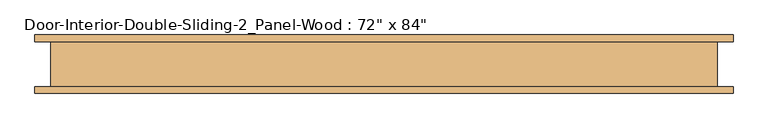
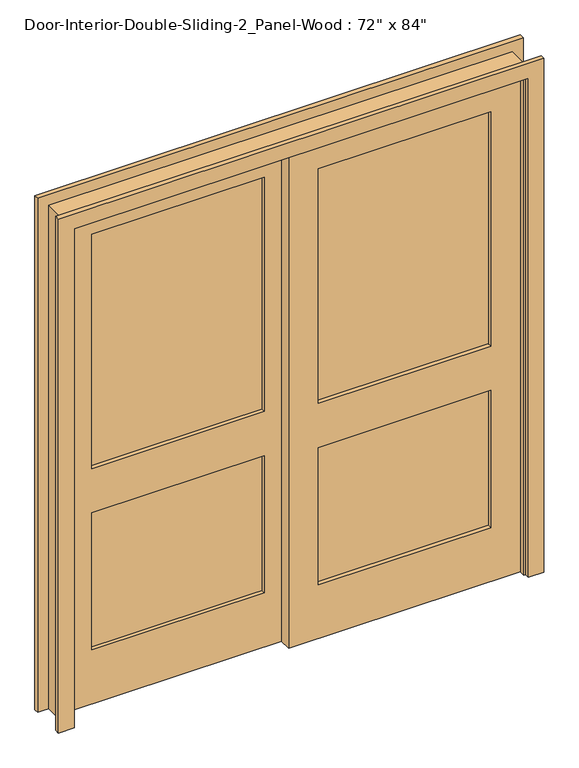
"""IFC4 building model written with IfcOpenShell, lengths in millimetres: door geometry."""

from ifc_helpers import new_model, si_unit, frame, origin, place, context, project, spatial, polyline, outline, extrude, source, transform, mapped, element, save


def door_029465dd(model_context):
    return source(origin(), model_context, "Body", "SweptSolid", [
        extrude(outline(polyline([(793.75, -24.3416667), (95.25, -24.3416667), (95.25, -7.4083333), (793.75, -7.4083333), (793.75, -24.3416667)])), frame((0.0, 0.0, 1009.65), z_axis=(0.0, 0.0, 1.0), x_axis=(1.0, 0.0, 0.0)), (0.0, 0.0, 1.0), 1004.8875),
        extrude(outline(polyline([(793.75, -24.3416667), (95.25, -24.3416667), (95.25, -7.4083333), (793.75, -7.4083333), (793.75, -24.3416667)])), frame((0.0, 0.0, 231.775), z_axis=(0.0, 0.0, 1.0), x_axis=(1.0, 0.0, 0.0)), (0.0, 0.0, 1.0), 587.375),
        extrude(outline(polyline([(2133.6, -25.4), (0.0, -25.4), (0.0, 914.4), (2133.6, 914.4), (2133.6, -25.4)]), holes=[polyline([(2014.5375, 95.25), (2014.5375, 793.75), (1009.65, 793.75), (1009.65, 95.25), (2014.5375, 95.25)]), polyline([(819.15, 95.25), (819.15, 793.75), (231.775, 793.75), (231.775, 95.25), (819.15, 95.25)])]), frame((0.0, -41.275, 0.0), z_axis=(0.0, 1.0, 0.0), x_axis=(0.0, 0.0, 1.0)), (0.0, 0.0, 1.0), 50.8),
        extrude(outline(polyline([(-95.25, 26.4583333), (-793.75, 26.4583333), (-793.75, 43.3916667), (-95.25, 43.3916667), (-95.25, 26.4583333)])), frame((0.0, 0.0, 1009.65), z_axis=(0.0, 0.0, 1.0), x_axis=(1.0, 0.0, 0.0)), (0.0, 0.0, 1.0), 1004.8875),
        extrude(outline(polyline([(-95.25, 26.4583333), (-793.75, 26.4583333), (-793.75, 43.3916667), (-95.25, 43.3916667), (-95.25, 26.4583333)])), frame((0.0, 0.0, 231.775), z_axis=(0.0, 0.0, 1.0), x_axis=(1.0, 0.0, 0.0)), (0.0, 0.0, 1.0), 587.375),
        extrude(outline(polyline([(2133.6, -914.4), (0.0, -914.4), (0.0, 25.4), (2133.6, 25.4), (2133.6, -914.4)]), holes=[polyline([(2014.5375, -793.75), (2014.5375, -95.25), (1009.65, -95.25), (1009.65, -793.75), (2014.5375, -793.75)]), polyline([(819.15, -793.75), (819.15, -95.25), (231.775, -95.25), (231.775, -793.75), (819.15, -793.75)])]), frame((0.0, 9.525, 0.0), z_axis=(0.0, 1.0, 0.0), x_axis=(0.0, 0.0, 1.0)), (0.0, 0.0, 1.0), 50.8),
        extrude(outline(polyline([(0.0, 914.4), (0.0, 939.8), (2159.0, 939.8), (2159.0, -939.8), (0.0, -939.8), (0.0, -914.4), (2133.6, -914.4), (2133.6, 914.4), (0.0, 914.4)])), frame((0.0, -66.675, 0.0), z_axis=(0.0, 1.0, 0.0), x_axis=(0.0, 0.0, 1.0)), (0.0, 0.0, 1.0), 127.0),
        extrude(outline(polyline([(0.0, 920.75), (0.0, 984.25), (2203.45, 984.25), (2203.45, -984.25), (0.0, -984.25), (0.0, -920.75), (2139.95, -920.75), (2139.95, 920.75), (0.0, 920.75)])), frame((0.0, -85.725, 0.0), z_axis=(0.0, 1.0, 0.0), x_axis=(0.0, 0.0, 1.0)), (0.0, 0.0, 1.0), 19.05),
        extrude(outline(polyline([(0.0, 920.75), (0.0, 984.25), (2203.45, 984.25), (2203.45, -984.25), (0.0, -984.25), (0.0, -920.75), (2139.95, -920.75), (2139.95, 920.75), (0.0, 920.75)])), frame((0.0, 60.325, 0.0), z_axis=(0.0, 1.0, 0.0), x_axis=(0.0, 0.0, 1.0)), (0.0, 0.0, 1.0), 19.05),
    ])


if __name__ == "__main__":
    model = new_model("IFC4")
    model_context = context("Model", 3, world=origin())
    ifc_project = project(units=[si_unit("LENGTHUNIT", "METRE", prefix="MILLI")], contexts=[model_context])
    site = spatial("IfcSite", under=ifc_project)
    building = spatial("IfcBuilding", under=site)
    placement = place(None, origin())
    door_shape = door_029465dd(model_context)
    element("IfcDoor", 1, ObjectType="Door-Interior-Double-Sliding-2_Panel-Wood : 72\" x 84\"", at=placement, inside=building, context=model_context, shape_type="MappedRepresentation", body=[
        mapped(door_shape, transform((0.0, 0.0, 0.0), x_axis=(1.0, 0.0, 0.0), y_axis=(0.0, 1.0, 0.0), z_axis=(0.0, 0.0, 1.0))),
    ])
    save(model, "model.ifc")

# Revit data of these elements
# Project information
#   Organization Name = "G3B Press"
#   Organization Description = "Paul F. Aubin Cosulting Services, Inc."
#   Building Name = "Revit Essentials for Architecture"
#   Author = "Paul F. Aubin"
#   Author Website = "https://www.paulaubin.com"
#   Copyright = "Copyright © 2020 Paul F Aubin, all rights reserved"
#   Project Issue Date = "8/1/2020"
#   Project Status = "Design Development"
#   Client Name = "Groups and Links"
#   Project Address = "Enter address here"
#   Project Name = "Hotel"
#   Project Number = "2020.06A"
# Type "Door-Interior-Double-Sliding-2_Panel-Wood : 72\" x 84\""
#   Type Mark = "8"
#   Assembly Code = "C1020"
#   Analytic Construction = "Wooden"
#   Top Rail = 0' - 4 11/16"
#   Thickness = 0' - 2"
#   Thermal Resistance (R) = 2.5876 (h·ft²·°F)/BTU
#   Stiles = 0' - 4 3/4"
#   Rough Width = 6' - 2"
#   Rough Height = 7' - 1"
#   Lock Rail = 0' - 7 1/2"
#   Heat Transfer Coefficient (U) = 0.3865 BTU/(h·ft²·°F)
#   Bottom Rail = 0' - 9 1/8"
#   Height = 7' - 0"
#   Width = 6' - 0"
#   Define Thermal Properties by = 1
#   Trim Material = Cherry
#   Panel Material = Cherry
#   Frame Material = Door - Frame
#   Visual Light Transmittance = 0
#   Solar Heat Gain Coefficient = 0
#   Function = (empty or 0)
#   Wall Closure = (empty or 0)
# Element 1 (IfcDoor, "Door-Interior-Double-Sliding-2_Panel-Wood : 72\" x 84\"")
#   Materials on its faces: "Cherry", "Door - Frame"
# Materials
#   "Cherry": class "Wood", colour RGB 157 77 38, transparency 0, Description = "Prunus Serotina", Cost = 0
#   "Door - Frame": class "Unassigned", colour RGB 118 70 51, transparency 0
